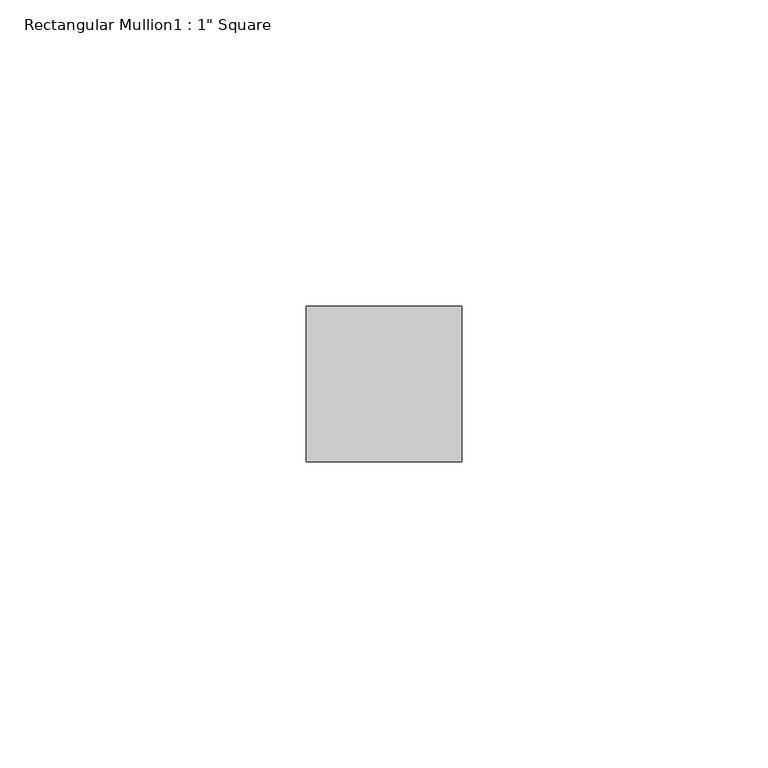
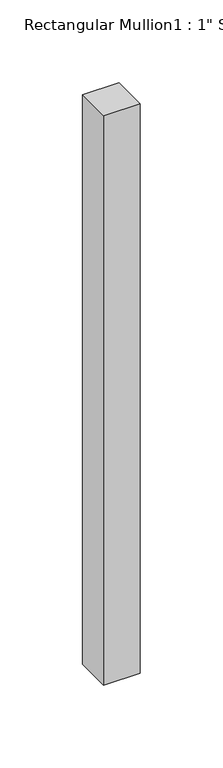
"""IFC4 building model written with IfcOpenShell, lengths in millimetres: member geometry."""

import ifcopenshell
import ifcopenshell.guid

model = None  # the IFC model being written
_history = None  # IfcOwnerHistory: only IFC2X3 demands one
_inside = {}  # id of a spatial element -> (the spatial element, [elements in it])
_under = {}  # id of a project, library or spatial element -> (it, [spatial elements below it])
_declared = {}  # id of a project -> (the project, [libraries it declares])
_typed = {}  # id of a type object -> (the type object, [elements of that type])
_made_of = {}  # id of a material, layer set ... -> (it, [elements and type objects made of it])


def new_model(schema):
    """Start an empty IFC model of exactly this schema.

    Asked for "IFC4X3", IfcOpenShell would pick the latest addendum, in which some entities
    have other attributes; the version numbers below select the first issue.
    IFC2X3 requires an IfcOwnerHistory on every rooted entity: one is made here for all.
    """
    global model, _history
    if schema == "IFC4X3":
        model = ifcopenshell.file(schema_version=(4, 3, 0, 0))
    else:
        model = ifcopenshell.file(schema=schema)
    _inside.clear()
    _under.clear()
    _declared.clear()
    _typed.clear()
    _made_of.clear()
    _history = None
    if model.schema == "IFC2X3":
        org = make("IfcOrganization", Name="unknown")
        user = make(
            "IfcPersonAndOrganization",
            ThePerson=make("IfcPerson", FamilyName="unknown"),
            TheOrganization=org,
        )
        app = make(
            "IfcApplication",
            ApplicationDeveloper=org,
            Version="unknown",
            ApplicationFullName="unknown",
            ApplicationIdentifier="unknown",
        )
        _history = make(
            "IfcOwnerHistory",
            OwningUser=user,
            OwningApplication=app,
            ChangeAction="ADDED",
            CreationDate=0,
        )
    return model


def make(cls, **values):
    """One entity of the class cls with the attributes given. An attribute that is None is left unset."""
    return model.create_entity(
        cls, **{name: value for name, value in values.items() if value is not None}
    )


def rooted(cls, **values):
    """An entity with a GlobalId (a new one), such as an element, a storey or a relation."""
    return make(cls, GlobalId=ifcopenshell.guid.new(), OwnerHistory=_history, **values)


def si_unit(unit_type, name, prefix=None):
    """IfcSIUnit, for example si_unit("LENGTHUNIT", "METRE", prefix="MILLI")."""
    return make("IfcSIUnit", UnitType=unit_type, Prefix=prefix, Name=name)


def assignment(units):
    """IfcUnitAssignment: the units of a project."""
    return None if units is None else make("IfcUnitAssignment", Units=units)


def point(xyz):
    """IfcCartesianPoint."""
    return None if xyz is None else make("IfcCartesianPoint", Coordinates=xyz)


def direction(xyz):
    """IfcDirection."""
    return None if xyz is None else make("IfcDirection", DirectionRatios=xyz)


def frame(location, z_axis=None, x_axis=None):
    """IfcAxis2Placement3D, a coordinate frame: its origin and axes. An axis left out is left unset."""
    return make(
        "IfcAxis2Placement3D",
        Location=point(location),
        Axis=direction(z_axis),
        RefDirection=direction(x_axis),
    )


def origin():
    """The frame at (0, 0, 0) with its axes left unset."""
    return frame((0.0, 0.0, 0.0))


def place(relative_to, where):
    """IfcLocalPlacement: puts the frame where relative to a parent placement (None: the world)."""
    return make(
        "IfcLocalPlacement", PlacementRelTo=relative_to, RelativePlacement=where
    )


def context(
    kind, dimensions, precision=None, world=None, true_north=None, identifier=None
):
    """IfcGeometricRepresentationContext, for example the 3D "Model" context."""
    return make(
        "IfcGeometricRepresentationContext",
        ContextIdentifier=identifier,
        ContextType=kind,
        CoordinateSpaceDimension=dimensions,
        Precision=precision,
        WorldCoordinateSystem=world,
        TrueNorth=true_north,
    )


def project(units=None, contexts=None):
    """IfcProject with its units and contexts."""
    return rooted(
        "IfcProject",
        Name="project",
        RepresentationContexts=contexts,
        UnitsInContext=assignment(units),
    )


def spatial(cls, under=None, at=None, **own):
    """A site, building, storey or space (cls), placed at a placement, below another one or the project."""
    s = rooted(cls, ObjectPlacement=at, **own)
    if under is not None:
        _under.setdefault(under.id(), (under, []))[1].append(s)
    return s


def polyline(points):
    """IfcPolyline through the points."""
    return make("IfcPolyline", Points=[point(p) for p in points])


def outline(outer, holes=None, kind="AREA"):
    """IfcArbitraryClosedProfileDef: a profile drawn as a closed curve; with holes, ...WithVoids."""
    if holes is None:
        return make("IfcArbitraryClosedProfileDef", ProfileType=kind, OuterCurve=outer)
    return make(
        "IfcArbitraryProfileDefWithVoids",
        ProfileType=kind,
        OuterCurve=outer,
        InnerCurves=holes,
    )


def extrude(swept, where, along, depth):
    """IfcExtrudedAreaSolid: the profile swept, set in the frame where, extruded along a direction by depth."""
    return make(
        "IfcExtrudedAreaSolid",
        SweptArea=swept,
        Position=where,
        ExtrudedDirection=direction(along),
        Depth=depth,
    )


def shape(context_of_items, identifier, shape_type, items):
    """IfcShapeRepresentation: the items that make up one representation, for example the "Body"."""
    return make(
        "IfcShapeRepresentation",
        ContextOfItems=context_of_items,
        RepresentationIdentifier=identifier,
        RepresentationType=shape_type,
        Items=items,
    )


def source(mapping_origin, context_of_items, identifier, shape_type, items):
    """IfcRepresentationMap: a shape defined once, which mapped items show again and again."""
    return make(
        "IfcRepresentationMap",
        MappingOrigin=mapping_origin,
        MappedRepresentation=shape(context_of_items, identifier, shape_type, items),
    )


def transform(
    local_origin,
    x_axis=None,
    y_axis=None,
    z_axis=None,
    scale=None,
    scale2=None,
    scale3=None,
    uniform=True,
):
    """IfcCartesianTransformationOperator3D, or its non-uniform kind. x_axis, y_axis, z_axis: its Axis1, 2, 3."""
    if uniform:
        return make(
            "IfcCartesianTransformationOperator3D",
            Axis1=direction(x_axis),
            Axis2=direction(y_axis),
            LocalOrigin=point(local_origin),
            Scale=scale,
            Axis3=direction(z_axis),
        )
    return make(
        "IfcCartesianTransformationOperator3DnonUniform",
        Axis1=direction(x_axis),
        Axis2=direction(y_axis),
        LocalOrigin=point(local_origin),
        Scale=scale,
        Axis3=direction(z_axis),
        Scale2=scale2,
        Scale3=scale3,
    )


def mapped(mapping_source, mapping_target):
    """IfcMappedItem: shows the shape of a source again, moved by a transform."""
    return make(
        "IfcMappedItem", MappingSource=mapping_source, MappingTarget=mapping_target
    )


def made_of(thing, what):
    """Note that an element or type object is made of a material, layer set ...; save() writes the relation."""
    if what is not None:
        _made_of.setdefault(what.id(), (what, []))[1].append(thing)
    return thing


def element(
    cls,
    number,
    at=None,
    inside=None,
    cuts=None,
    type_object=None,
    material=None,
    context=None,
    identifier="Body",
    shape_type=None,
    held_by="IfcProductDefinitionShape",
    body=None,
    shapes=None,
    **own,
):
    """One element of the class cls, such as IfcWall. Its Tag is "e" and its number.

    at: its placement. inside: the storey or other place that contains it. cuts: it is an
    opening in that element (IfcRelVoidsElement). A single representation is given by context,
    identifier, shape_type and body (its items); several are given by shapes. held_by: the class
    of the entity that holds the representations. save() writes the other relations.
    """
    e = rooted(cls, Tag="e%d" % number, ObjectPlacement=at, **own)
    if body is not None:
        shapes = [shape(context, identifier, shape_type, body)]
    if shapes is not None:
        e.Representation = make(held_by, Representations=shapes)
    if inside is not None:
        _inside.setdefault(inside.id(), (inside, []))[1].append(e)
    if cuts is not None:
        rooted(
            "IfcRelVoidsElement", RelatingBuildingElement=cuts, RelatedOpeningElement=e
        )
    if type_object is not None:
        _typed.setdefault(type_object.id(), (type_object, []))[1].append(e)
    return made_of(e, material)


def aggregate(whole, parts):
    """IfcRelAggregates: a whole, such as a stair, and the parts it consists of."""
    return rooted("IfcRelAggregates", RelatingObject=whole, RelatedObjects=parts)


def save(model, path):
    """Write the relations noted so far, then the file.

    IfcRelAggregates (storeys below a building ...), IfcRelContainedInSpatialStructure (elements
    in a storey), IfcRelDefinesByType, IfcRelAssociatesMaterial and IfcRelDeclares: one each for
    every whole, place, type object, material and project.
    """
    for whole, parts in _under.values():
        aggregate(whole, parts)
    for where, things in _inside.values():
        rooted(
            "IfcRelContainedInSpatialStructure",
            RelatedElements=things,
            RelatingStructure=where,
        )
    for kind, things in _typed.values():
        rooted("IfcRelDefinesByType", RelatedObjects=things, RelatingType=kind)
    for what, things in _made_of.values():
        rooted("IfcRelAssociatesMaterial", RelatedObjects=things, RelatingMaterial=what)
    for by, libraries in _declared.values():
        rooted("IfcRelDeclares", RelatingContext=by, RelatedDefinitions=libraries)
    model.write(path)


def member_efb85692(model_context):
    return source(origin(), model_context, "Body", "SweptSolid", [
        extrude(outline(polyline([(12.7, -19.05), (12.7, -44.45), (-12.7, -44.45), (-12.7, -19.05), (12.7, -19.05)])), frame((0.0, 0.0, -419.1), z_axis=(0.0, 0.0, 1.0), x_axis=(1.0, 0.0, 0.0)), (0.0, 0.0, 1.0), 419.1),
    ])


if __name__ == "__main__":
    model = new_model("IFC4")
    model_context = context("Model", 3, world=origin())
    ifc_project = project(units=[si_unit("LENGTHUNIT", "METRE", prefix="MILLI")], contexts=[model_context])
    site = spatial("IfcSite", under=ifc_project)
    building = spatial("IfcBuilding", under=site)
    placement = place(None, origin())
    member_shape = member_efb85692(model_context)
    element("IfcMember", 1, ObjectType="Rectangular Mullion1 : 1\" Square", at=placement, inside=building, context=model_context, shape_type="MappedRepresentation", body=[
        mapped(member_shape, transform((0.0, 0.0, 0.0), x_axis=(1.0, 0.0, 0.0), y_axis=(0.0, 1.0, 0.0), z_axis=(0.0, 0.0, 1.0))),
    ])
    save(model, "model.ifc")

# Revit data of these elements
# Type "Rectangular Mullion1 : 1\" Square"
#   built-in parameter 1007351 = 0.104167 (stored number, unit not read)
#   built-in parameter 1007304 = 0.0833333 (stored number, unit not read)
#   built-in parameter 1007301 = 0.0416667 (stored number, unit not read)
#   built-in parameter 1007300 = 0.0416667 (stored number, unit not read)
